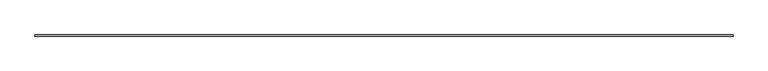
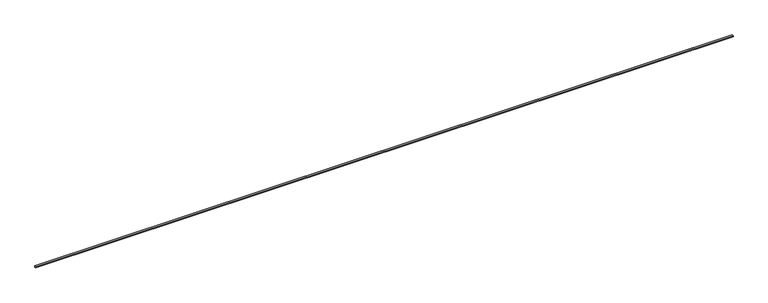
"""IFC4 building model written with IfcOpenShell, lengths in millimetres: proxy geometry, Joint003 2207 : Joint003 2207."""

from ifc_helpers import new_model, si_unit, point, frame, frame_2d, origin, place, context, project, spatial, polyline, circle_curve, trimmed, segment, composite_curve, outline, extrude, source, transform, mapped, element, save


def generic_models_62c951ce(model_context):
    return source(origin(), model_context, "Body", "SweptSolid", [
        extrude(outline(composite_curve([segment(polyline([(9721.6885026, 39515.7608438), (9721.6885026, 39511.842875)]), True, "CONTINUOUS"), segment(trimmed(circle_curve(frame_2d((9720.0901706, 39506.671)), 5.4132205), [point((9721.6885026, 39511.842875))], [point((9718.4918386, 39511.842875))], True, "CARTESIAN"), True, "CONTINUOUS"), segment(polyline([(9718.4918386, 39511.842875), (9718.4918386, 39515.7608438)]), True, "CONTINUOUS"), segment(trimmed(circle_curve(frame_2d((9720.0901706, 39510.5889688)), 5.4132205), [point((9718.4918386, 39515.7608438))], [point((9721.6885026, 39515.7608438))], False, "CARTESIAN"), True, "CONTINUOUS")], self_intersect=False)), frame((3694.2883192, 0.0, 0.0), z_axis=(1.0, 0.0, 0.0), x_axis=(0.0, 1.0, 0.0)), (0.0, 0.0, 1.0), 2000.0),
    ])


if __name__ == "__main__":
    model = new_model("IFC4")
    model_context = context("Model", 3, world=origin())
    ifc_project = project(units=[si_unit("LENGTHUNIT", "METRE", prefix="MILLI")], contexts=[model_context])
    site = spatial("IfcSite", under=ifc_project)
    building = spatial("IfcBuilding", under=site)
    placement = place(None, origin())
    generic_models_shape = generic_models_62c951ce(model_context)
    element("IfcBuildingElementProxy", 1, Name="Joint003 2207 : Joint003 2207", ObjectType="Joint003 2207 : Joint003 2207", at=placement, inside=building, context=model_context, shape_type="MappedRepresentation", body=[
        mapped(generic_models_shape, transform((0.0, 0.0, 0.0), x_axis=(1.0, 0.0, 0.0), y_axis=(0.0, 1.0, 0.0), z_axis=(0.0, 0.0, 1.0))),
    ])
    save(model, "model.ifc")

# Revit data of these elements
# Type "Joint003 2207 : Joint003 2207"
#   NameOverride = "Joint003"
# Element 1 (IfcBuildingElementProxy, "Joint003 2207 : Joint003 2207")
#   Materials on its faces: "SILICON JOINT"
# Materials
#   "SILICON JOINT": class "Unassigned", colour RGB 150 184 127, transparency 0
